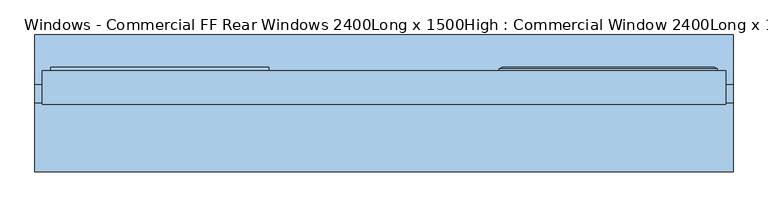
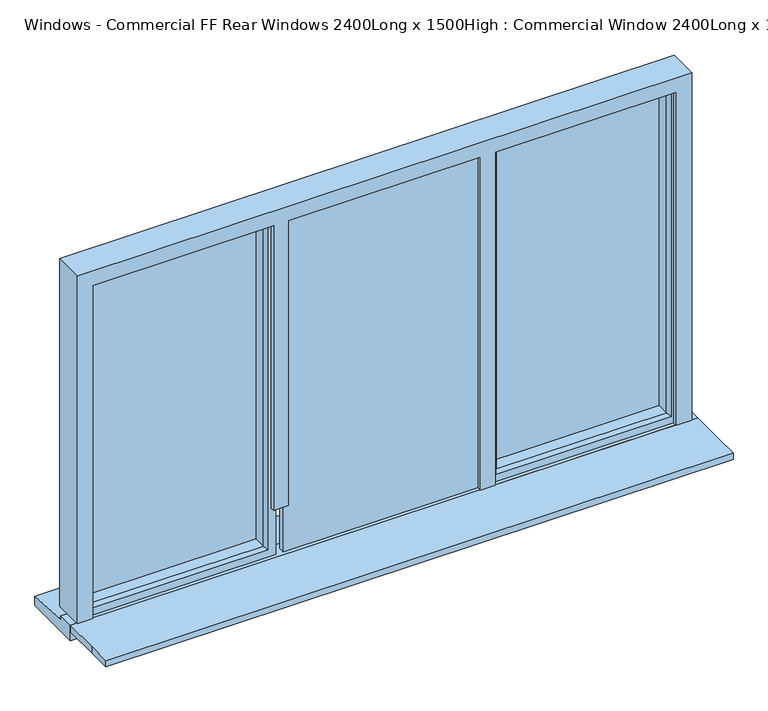
"""IFC4 building model written with IfcOpenShell, lengths in millimetres: window geometry, Windows - Commercial FF Rear Windows 2400Long x 1500High : Commercial Window 2400Long x 1500High."""

import ifcopenshell
import ifcopenshell.guid

model = None  # the IFC model being written
_history = None  # IfcOwnerHistory: only IFC2X3 demands one
_inside = {}  # id of a spatial element -> (the spatial element, [elements in it])
_under = {}  # id of a project, library or spatial element -> (it, [spatial elements below it])
_declared = {}  # id of a project -> (the project, [libraries it declares])
_typed = {}  # id of a type object -> (the type object, [elements of that type])
_made_of = {}  # id of a material, layer set ... -> (it, [elements and type objects made of it])


def new_model(schema):
    """Start an empty IFC model of exactly this schema.

    Asked for "IFC4X3", IfcOpenShell would pick the latest addendum, in which some entities
    have other attributes; the version numbers below select the first issue.
    IFC2X3 requires an IfcOwnerHistory on every rooted entity: one is made here for all.
    """
    global model, _history
    if schema == "IFC4X3":
        model = ifcopenshell.file(schema_version=(4, 3, 0, 0))
    else:
        model = ifcopenshell.file(schema=schema)
    _inside.clear()
    _under.clear()
    _declared.clear()
    _typed.clear()
    _made_of.clear()
    _history = None
    if model.schema == "IFC2X3":
        org = make("IfcOrganization", Name="unknown")
        user = make(
            "IfcPersonAndOrganization",
            ThePerson=make("IfcPerson", FamilyName="unknown"),
            TheOrganization=org,
        )
        app = make(
            "IfcApplication",
            ApplicationDeveloper=org,
            Version="unknown",
            ApplicationFullName="unknown",
            ApplicationIdentifier="unknown",
        )
        _history = make(
            "IfcOwnerHistory",
            OwningUser=user,
            OwningApplication=app,
            ChangeAction="ADDED",
            CreationDate=0,
        )
    return model


def make(cls, **values):
    """One entity of the class cls with the attributes given. An attribute that is None is left unset."""
    return model.create_entity(
        cls, **{name: value for name, value in values.items() if value is not None}
    )


def rooted(cls, **values):
    """An entity with a GlobalId (a new one), such as an element, a storey or a relation."""
    return make(cls, GlobalId=ifcopenshell.guid.new(), OwnerHistory=_history, **values)


def si_unit(unit_type, name, prefix=None):
    """IfcSIUnit, for example si_unit("LENGTHUNIT", "METRE", prefix="MILLI")."""
    return make("IfcSIUnit", UnitType=unit_type, Prefix=prefix, Name=name)


def assignment(units):
    """IfcUnitAssignment: the units of a project."""
    return None if units is None else make("IfcUnitAssignment", Units=units)


def point(xyz):
    """IfcCartesianPoint."""
    return None if xyz is None else make("IfcCartesianPoint", Coordinates=xyz)


def direction(xyz):
    """IfcDirection."""
    return None if xyz is None else make("IfcDirection", DirectionRatios=xyz)


def frame(location, z_axis=None, x_axis=None):
    """IfcAxis2Placement3D, a coordinate frame: its origin and axes. An axis left out is left unset."""
    return make(
        "IfcAxis2Placement3D",
        Location=point(location),
        Axis=direction(z_axis),
        RefDirection=direction(x_axis),
    )


def origin():
    """The frame at (0, 0, 0) with its axes left unset."""
    return frame((0.0, 0.0, 0.0))


def place(relative_to, where):
    """IfcLocalPlacement: puts the frame where relative to a parent placement (None: the world)."""
    return make(
        "IfcLocalPlacement", PlacementRelTo=relative_to, RelativePlacement=where
    )


def context(
    kind, dimensions, precision=None, world=None, true_north=None, identifier=None
):
    """IfcGeometricRepresentationContext, for example the 3D "Model" context."""
    return make(
        "IfcGeometricRepresentationContext",
        ContextIdentifier=identifier,
        ContextType=kind,
        CoordinateSpaceDimension=dimensions,
        Precision=precision,
        WorldCoordinateSystem=world,
        TrueNorth=true_north,
    )


def project(units=None, contexts=None):
    """IfcProject with its units and contexts."""
    return rooted(
        "IfcProject",
        Name="project",
        RepresentationContexts=contexts,
        UnitsInContext=assignment(units),
    )


def spatial(cls, under=None, at=None, **own):
    """A site, building, storey or space (cls), placed at a placement, below another one or the project."""
    s = rooted(cls, ObjectPlacement=at, **own)
    if under is not None:
        _under.setdefault(under.id(), (under, []))[1].append(s)
    return s


def polyline(points):
    """IfcPolyline through the points."""
    return make("IfcPolyline", Points=[point(p) for p in points])


def outline(outer, holes=None, kind="AREA"):
    """IfcArbitraryClosedProfileDef: a profile drawn as a closed curve; with holes, ...WithVoids."""
    if holes is None:
        return make("IfcArbitraryClosedProfileDef", ProfileType=kind, OuterCurve=outer)
    return make(
        "IfcArbitraryProfileDefWithVoids",
        ProfileType=kind,
        OuterCurve=outer,
        InnerCurves=holes,
    )


def extrude(swept, where, along, depth):
    """IfcExtrudedAreaSolid: the profile swept, set in the frame where, extruded along a direction by depth."""
    return make(
        "IfcExtrudedAreaSolid",
        SweptArea=swept,
        Position=where,
        ExtrudedDirection=direction(along),
        Depth=depth,
    )


def faces_of(points, faces, orient=None, outer=None):
    """IfcFace entities. A face is a list of loops; a loop is a list of indices into points, from 0.

    orient and outer hold one flag for each loop. By default every Orientation is true, the
    first loop of a face is its IfcFaceOuterBound and the others are IfcFaceBound.
    """
    made = []
    for i, loops in enumerate(faces):
        bounds = []
        for j, loop in enumerate(loops):
            is_outer = j == 0 if outer is None else outer[i][j]
            bounds.append(
                make(
                    "IfcFaceOuterBound" if is_outer else "IfcFaceBound",
                    Bound=make("IfcPolyLoop", Polygon=[points[k] for k in loop]),
                    Orientation=True if orient is None else orient[i][j],
                )
            )
        made.append(make("IfcFace", Bounds=bounds))
    return made


def faceted_brep(points, faces, orient=None, outer=None, voids=None):
    """IfcFacetedBrep: a solid bounded by flat faces; with voids (closed shells), ...WithVoids."""
    shared = [point(p) for p in points]
    hull = make("IfcClosedShell", CfsFaces=faces_of(shared, faces, orient, outer))
    if voids is None:
        return make("IfcFacetedBrep", Outer=hull)
    return make(
        "IfcFacetedBrepWithVoids",
        Outer=hull,
        Voids=[
            make(cls, CfsFaces=faces_of(shared, fs, o, b)) for cls, fs, o, b in voids
        ],
    )


def shape(context_of_items, identifier, shape_type, items):
    """IfcShapeRepresentation: the items that make up one representation, for example the "Body"."""
    return make(
        "IfcShapeRepresentation",
        ContextOfItems=context_of_items,
        RepresentationIdentifier=identifier,
        RepresentationType=shape_type,
        Items=items,
    )


def source(mapping_origin, context_of_items, identifier, shape_type, items):
    """IfcRepresentationMap: a shape defined once, which mapped items show again and again."""
    return make(
        "IfcRepresentationMap",
        MappingOrigin=mapping_origin,
        MappedRepresentation=shape(context_of_items, identifier, shape_type, items),
    )


def transform(
    local_origin,
    x_axis=None,
    y_axis=None,
    z_axis=None,
    scale=None,
    scale2=None,
    scale3=None,
    uniform=True,
):
    """IfcCartesianTransformationOperator3D, or its non-uniform kind. x_axis, y_axis, z_axis: its Axis1, 2, 3."""
    if uniform:
        return make(
            "IfcCartesianTransformationOperator3D",
            Axis1=direction(x_axis),
            Axis2=direction(y_axis),
            LocalOrigin=point(local_origin),
            Scale=scale,
            Axis3=direction(z_axis),
        )
    return make(
        "IfcCartesianTransformationOperator3DnonUniform",
        Axis1=direction(x_axis),
        Axis2=direction(y_axis),
        LocalOrigin=point(local_origin),
        Scale=scale,
        Axis3=direction(z_axis),
        Scale2=scale2,
        Scale3=scale3,
    )


def mapped(mapping_source, mapping_target):
    """IfcMappedItem: shows the shape of a source again, moved by a transform."""
    return make(
        "IfcMappedItem", MappingSource=mapping_source, MappingTarget=mapping_target
    )


def made_of(thing, what):
    """Note that an element or type object is made of a material, layer set ...; save() writes the relation."""
    if what is not None:
        _made_of.setdefault(what.id(), (what, []))[1].append(thing)
    return thing


def element(
    cls,
    number,
    at=None,
    inside=None,
    cuts=None,
    type_object=None,
    material=None,
    context=None,
    identifier="Body",
    shape_type=None,
    held_by="IfcProductDefinitionShape",
    body=None,
    shapes=None,
    **own,
):
    """One element of the class cls, such as IfcWall. Its Tag is "e" and its number.

    at: its placement. inside: the storey or other place that contains it. cuts: it is an
    opening in that element (IfcRelVoidsElement). A single representation is given by context,
    identifier, shape_type and body (its items); several are given by shapes. held_by: the class
    of the entity that holds the representations. save() writes the other relations.
    """
    e = rooted(cls, Tag="e%d" % number, ObjectPlacement=at, **own)
    if body is not None:
        shapes = [shape(context, identifier, shape_type, body)]
    if shapes is not None:
        e.Representation = make(held_by, Representations=shapes)
    if inside is not None:
        _inside.setdefault(inside.id(), (inside, []))[1].append(e)
    if cuts is not None:
        rooted(
            "IfcRelVoidsElement", RelatingBuildingElement=cuts, RelatedOpeningElement=e
        )
    if type_object is not None:
        _typed.setdefault(type_object.id(), (type_object, []))[1].append(e)
    return made_of(e, material)


def aggregate(whole, parts):
    """IfcRelAggregates: a whole, such as a stair, and the parts it consists of."""
    return rooted("IfcRelAggregates", RelatingObject=whole, RelatedObjects=parts)


def save(model, path):
    """Write the relations noted so far, then the file.

    IfcRelAggregates (storeys below a building ...), IfcRelContainedInSpatialStructure (elements
    in a storey), IfcRelDefinesByType, IfcRelAssociatesMaterial and IfcRelDeclares: one each for
    every whole, place, type object, material and project.
    """
    for whole, parts in _under.values():
        aggregate(whole, parts)
    for where, things in _inside.values():
        rooted(
            "IfcRelContainedInSpatialStructure",
            RelatedElements=things,
            RelatingStructure=where,
        )
    for kind, things in _typed.values():
        rooted("IfcRelDefinesByType", RelatedObjects=things, RelatingType=kind)
    for what, things in _made_of.values():
        rooted("IfcRelAssociatesMaterial", RelatedObjects=things, RelatingMaterial=what)
    for by, libraries in _declared.values():
        rooted("IfcRelDeclares", RelatingContext=by, RelatedDefinitions=libraries)
    model.write(path)


def windows_commercial_ff_rear_windows_2400long_x_1500high_d88e899e(model_context):
    return source(origin(), model_context, "Body", "SolidModel", [
        extrude(outline(polyline([(-1860.0, -231.5434322), (-1860.0, -138.5434322), (-1860.0, 8.4565678), (590.0, 8.4565678), (590.0, -138.5434322), (590.0, -231.5434322), (-1860.0, -231.5434322)])), frame((0.0, 0.0, 636.5715519), z_axis=(0.0, 0.0, 1.0), x_axis=(1.0, 0.0, 0.0)), (0.0, 0.0, 1.0), 26.4284481),
        extrude(outline(polyline([(495.0, 87.4565678), (-190.0, 87.4565678), (-190.0, 111.4565678), (495.0, 111.4565678), (495.0, 87.4565678)])), frame((0.0, 0.0, 693.0), z_axis=(0.0, 0.0, 1.0), x_axis=(1.0, 0.0, 0.0)), (0.0, 0.0, 1.0), 1337.0),
        extrude(outline(polyline([(-1020.0, 47.4565678), (-250.0, 47.4565678), (-250.0, 23.4565678), (-1020.0, 23.4565678), (-1020.0, 47.4565678)])), frame((0.0, 0.0, 663.0), z_axis=(0.0, 0.0, 1.0), x_axis=(1.0, 0.0, 0.0)), (0.0, 0.0, 1.0), 1397.0),
        extrude(outline(polyline([(-1080.0, 87.4565678), (-1765.0, 87.4565678), (-1765.0, 111.4565678), (-1080.0, 111.4565678), (-1080.0, 87.4565678)])), frame((0.0, 0.0, 693.0), z_axis=(0.0, 0.0, 1.0), x_axis=(1.0, 0.0, 0.0)), (0.0, 0.0, 1.0), 1337.0),
        faceted_brep([(-1835.0, 5.4565678, 663.0), (-1775.0, 5.4565678, 663.0), (-1775.0, 5.4565678, 2040.0), (-1068.0, 5.4565678, 2040.0), (-1068.0, 5.4565678, 863.0), (-1010.0, 5.4565678, 863.0), (-1010.0, 5.4565678, 2040.0), (-260.0, 5.4565678, 2040.0), (-260.0, 5.4565678, 663.0), (-202.0, 5.4565678, 663.0), (-202.0, 5.4565678, 2040.0), (505.0, 5.4565678, 2040.0), (505.0, 5.4565678, 663.0), (565.0, 5.4565678, 663.0), (565.0, 5.4565678, 2100.0), (-1835.0, 5.4565678, 2100.0), (-1835.0, 123.4565678, 2100.0), (-1835.0, 123.4565678, 663.0), (-1835.0, 73.4565678, 663.0), (-1835.0, 8.4565678, 663.0), (-1795.0, 123.4565678, 663.0), (565.0, 123.4565678, 2100.0), (565.0, 123.4565678, 663.0), (525.0, 123.4565678, 663.0), (525.0, 123.4565678, 2060.0), (-220.0, 123.4565678, 2060.0), (-220.0, 123.4565678, 663.0), (-260.0, 123.4565678, 663.0), (-260.0, 123.4565678, 2060.0), (-1010.0, 123.4565678, 2060.0), (-1010.0, 123.4565678, 863.0), (-1050.0, 123.4565678, 863.0), (-1050.0, 123.4565678, 2060.0), (-1795.0, 123.4565678, 2060.0), (-1795.0, 23.4565678, 2060.0), (-1795.0, 23.4565678, 663.0), (-1795.0, 73.4565678, 663.0), (-1050.0, 23.4565678, 2060.0), (-1050.0, 23.4565678, 863.0), (-1068.0, 23.4565678, 863.0), (-1068.0, 23.4565678, 2040.0), (-1775.0, 23.4565678, 2040.0), (-1775.0, 23.4565678, 663.0), (525.0, 23.4565678, 2060.0), (525.0, 23.4565678, 663.0), (505.0, 23.4565678, 663.0), (505.0, 23.4565678, 2040.0), (-202.0, 23.4565678, 2040.0), (-202.0, 23.4565678, 663.0), (-220.0, 23.4565678, 663.0), (-220.0, 23.4565678, 2060.0), (-1010.0, 23.4565678, 863.0), (-1020.0, 23.4565678, 863.0), (-1020.0, 23.4565678, 2060.0), (-250.0, 23.4565678, 2060.0), (-250.0, 23.4565678, 663.0), (-260.0, 23.4565678, 663.0), (-260.0, 23.4565678, 2040.0), (-1010.0, 23.4565678, 2040.0), (-1775.0, 8.4565678, 663.0), (-1010.0, 47.4565678, 2060.0), (-260.0, 47.4565678, 2060.0), (-250.0, 47.4565678, 2060.0), (-1020.0, 47.4565678, 2060.0), (565.0, 8.4565678, 663.0), (565.0, 73.4565678, 663.0), (525.0, 73.4565678, 663.0), (505.0, 8.4565678, 663.0), (-1010.0, 47.4565678, 863.0), (-1020.0, 47.4565678, 863.0), (-250.0, 47.4565678, 663.0), (-260.0, 47.4565678, 663.0), (-260.0, 73.4565678, 663.0), (-220.0, 73.4565678, 663.0), (-202.0, 8.4565678, 663.0), (-260.0, 8.4565678, 663.0), (590.0, 248.4565678, 600.0), (590.0, 8.4565678, 600.0), (-1860.0, 8.4565678, 600.0), (-1860.0, 248.4565678, 600.0), (590.0, 248.4565678, 637.0666405), (-1860.0, 248.4565678, 637.0666405), (590.0, 73.4565678, 649.0962075), (-1860.0, 73.4565678, 649.0962075), (590.0, 8.4565678, 663.0), (590.0, 73.4565678, 663.0), (-1860.0, 73.4565678, 663.0), (-1860.0, 8.4565678, 663.0)], [[[0, 1, 2, 3, 4, 5, 6, 7, 8, 9, 10, 11, 12, 13, 14, 15]], [[0, 15, 16, 17, 18, 19]], [[20, 17, 16, 21, 22, 23, 24, 25, 26, 27, 28, 29, 30, 31, 32, 33]], [[20, 33, 34, 35, 36]], [[35, 34, 37, 38, 39, 40, 41, 42]], [[43, 44, 45, 46, 47, 48, 49, 50]], [[51, 52, 53, 54, 55, 56, 57, 58]], [[2, 1, 59, 42, 41]], [[15, 14, 21, 16]], [[34, 33, 32, 37]], [[24, 43, 50, 25]], [[60, 29, 28, 61, 62, 54, 53, 63]], [[2, 41, 40, 3]], [[46, 11, 10, 47]], [[6, 58, 57, 7]], [[14, 13, 64, 65, 22, 21]], [[24, 23, 66, 44, 43]], [[12, 11, 46, 45, 67]], [[5, 51, 58, 6]], [[39, 4, 3, 40]], [[31, 38, 37, 32]], [[68, 30, 29, 60]], [[69, 68, 60, 63]], [[52, 69, 63, 53]], [[62, 70, 55, 54]], [[70, 62, 61, 71]], [[71, 61, 28, 27, 72]], [[26, 25, 50, 49, 73]], [[10, 9, 74, 48, 47]], [[8, 7, 57, 56, 75]], [[76, 77, 78, 79]], [[80, 76, 79, 81]], [[82, 80, 81, 83]], [[84, 85, 65, 64]], [[86, 87, 19, 18]], [[72, 36, 35, 42, 59, 75, 56, 55, 70, 71]], [[66, 73, 49, 48, 74, 67, 45, 44]], [[17, 20, 36, 18]], [[1, 0, 19, 59]], [[23, 22, 65, 66]], [[13, 12, 67, 64]], [[51, 5, 4, 39, 38, 31, 30, 68, 69, 52]], [[27, 26, 73, 72]], [[9, 8, 75, 74]], [[84, 77, 76, 80, 82, 85]], [[87, 86, 83, 81, 79, 78]], [[85, 82, 83, 86, 18, 36, 72, 73, 66, 65]], [[77, 84, 64, 67, 74, 75, 59, 19, 87, 78]]]),
        faceted_brep([(-1050.0, 23.4565678, 2060.0), (-1050.0, 93.4565678, 2060.0), (-1795.0, 93.4565678, 2060.0), (-1795.0, 23.4565678, 2060.0), (-1090.0, 37.9494677, 2020.0), (-1079.8519623, 23.4565678, 2030.1480377), (-1765.1480377, 23.4565678, 2030.1480377), (-1755.0, 37.9494677, 2020.0), (-1090.0, 87.4565678, 2020.0), (-1755.0, 87.4565678, 2020.0), (-1080.0, 111.4565678, 2030.0), (-1080.0, 87.4565678, 2030.0), (-1765.0, 87.4565678, 2030.0), (-1765.0, 111.4565678, 2030.0), (-1090.0, 129.2300705, 2020.0), (-1090.0, 111.4565678, 2020.0), (-1755.0, 111.4565678, 2020.0), (-1755.0, 129.2300705, 2020.0), (-1071.1854344, 135.0035732, 2038.8145656), (-1773.8145656, 135.0035732, 2038.8145656), (-1795.0, 93.4565678, 663.0), (-1795.0, 23.4565678, 663.0), (-1765.1480377, 23.4565678, 692.8519623), (-1755.0, 37.9494677, 703.0), (-1755.0, 87.4565678, 703.0), (-1765.0, 87.4565678, 693.0), (-1765.0, 111.4565678, 693.0), (-1755.0, 111.4565678, 703.0), (-1755.0, 129.2300705, 703.0), (-1773.8145656, 135.0035732, 684.1854344), (-1050.0, 93.4565678, 663.0), (-1050.0, 23.4565678, 663.0), (-1079.8519623, 23.4565678, 692.8519623), (-1090.0, 37.9494677, 703.0), (-1090.0, 87.4565678, 703.0), (-1080.0, 87.4565678, 693.0), (-1080.0, 111.4565678, 693.0), (-1090.0, 111.4565678, 703.0), (-1090.0, 129.2300705, 703.0), (-1071.1854344, 135.0035732, 684.1854344), (-1040.0, 135.0035732, 653.0), (-1805.0, 135.0035732, 653.0), (-1805.0, 135.0035732, 2070.0), (-1040.0, 135.0035732, 2070.0), (-1040.0, 93.4565678, 2070.0), (-1805.0, 93.4565678, 2070.0), (-1805.0, 93.4565678, 653.0), (-1040.0, 93.4565678, 653.0)], [[[0, 1, 2, 3]], [[4, 5, 6, 7]], [[8, 4, 7, 9]], [[10, 11, 12, 13]], [[14, 15, 16, 17]], [[18, 14, 17, 19]], [[3, 2, 20, 21]], [[7, 6, 22, 23]], [[9, 7, 23, 24]], [[13, 12, 25, 26]], [[17, 16, 27, 28]], [[19, 17, 28, 29]], [[21, 20, 30, 31]], [[0, 3, 21, 31], [32, 22, 6, 5]], [[23, 22, 32, 33]], [[24, 23, 33, 34]], [[35, 25, 12, 11], [8, 9, 24, 34]], [[26, 25, 35, 36]], [[10, 13, 26, 36], [37, 27, 16, 15]], [[28, 27, 37, 38]], [[29, 28, 38, 39]], [[40, 41, 42, 43], [18, 19, 29, 39]], [[30, 1, 0, 31]], [[33, 32, 5, 4]], [[34, 33, 4, 8]], [[36, 35, 11, 10]], [[38, 37, 15, 14]], [[39, 38, 14, 18]], [[44, 43, 42, 45]], [[45, 42, 41, 46]], [[46, 41, 40, 47]], [[47, 40, 43, 44]], [[45, 46, 47, 44], [1, 30, 20, 2]]]),
        faceted_brep([(-230.0, 87.4565678, 2070.0), (-230.0, 129.2300705, 2070.0), (-230.0, 129.2300705, 653.0), (-230.0, 87.4565678, 653.0), (-220.0, 23.4565678, 2060.0), (-220.0, 87.4565678, 2060.0), (-220.0, 87.4565678, 663.0), (-220.0, 23.4565678, 663.0), (-180.0, 37.9494677, 2020.0), (-190.1480377, 23.4565678, 2030.1480377), (-190.1480377, 23.4565678, 692.8519623), (-180.0, 37.9494677, 703.0), (-180.0, 87.4565678, 2020.0), (-180.0, 87.4565678, 703.0), (-190.0, 111.4565678, 2030.0), (-190.0, 87.4565678, 2030.0), (-190.0, 87.4565678, 693.0), (-190.0, 111.4565678, 693.0), (-180.0, 129.2300705, 2020.0), (-180.0, 111.4565678, 2020.0), (-180.0, 111.4565678, 703.0), (-180.0, 129.2300705, 703.0), (-197.4457548, 135.0035732, 2037.4457548), (-197.4457548, 135.0035732, 685.5542452), (-219.2153903, 135.0035732, 2059.2153903), (-219.2153903, 135.0035732, 663.7846097), (535.0, 129.2300705, 653.0), (535.0, 87.4565678, 653.0), (525.0, 87.4565678, 663.0), (525.0, 23.4565678, 663.0), (495.1480377, 23.4565678, 692.8519623), (485.0, 37.9494677, 703.0), (485.0, 87.4565678, 703.0), (495.0, 87.4565678, 693.0), (495.0, 111.4565678, 693.0), (485.0, 111.4565678, 703.0), (485.0, 129.2300705, 703.0), (502.4457548, 135.0035732, 685.5542452), (524.2153903, 135.0035732, 663.7846097), (535.0, 129.2300705, 2070.0), (535.0, 87.4565678, 2070.0), (525.0, 87.4565678, 2060.0), (525.0, 23.4565678, 2060.0), (495.1480377, 23.4565678, 2030.1480377), (485.0, 37.9494677, 2020.0), (485.0, 87.4565678, 2020.0), (495.0, 87.4565678, 2030.0), (495.0, 111.4565678, 2030.0), (485.0, 111.4565678, 2020.0), (485.0, 129.2300705, 2020.0), (502.4457548, 135.0035732, 2037.4457548), (524.2153903, 135.0035732, 2059.2153903)], [[[0, 1, 2, 3]], [[4, 5, 6, 7]], [[8, 9, 10, 11]], [[12, 8, 11, 13]], [[14, 15, 16, 17]], [[18, 19, 20, 21]], [[22, 18, 21, 23]], [[1, 24, 25, 2]], [[3, 2, 26, 27]], [[7, 6, 28, 29]], [[11, 10, 30, 31]], [[13, 11, 31, 32]], [[17, 16, 33, 34]], [[21, 20, 35, 36]], [[23, 21, 36, 37]], [[2, 25, 38, 26]], [[27, 26, 39, 40]], [[29, 28, 41, 42]], [[31, 30, 43, 44]], [[32, 31, 44, 45]], [[34, 33, 46, 47]], [[36, 35, 48, 49]], [[37, 36, 49, 50]], [[26, 38, 51, 39]], [[40, 39, 1, 0]], [[42, 41, 5, 4]], [[7, 29, 42, 4], [9, 43, 30, 10]], [[44, 43, 9, 8]], [[45, 44, 8, 12]], [[15, 46, 33, 16], [13, 32, 45, 12]], [[47, 46, 15, 14]], [[17, 34, 47, 14], [19, 48, 35, 20]], [[49, 48, 19, 18]], [[50, 49, 18, 22]], [[24, 51, 38, 25], [23, 37, 50, 22]], [[39, 51, 24, 1]], [[3, 27, 40, 0], [5, 41, 28, 6]]]),
    ])


if __name__ == "__main__":
    model = new_model("IFC4")
    model_context = context("Model", 3, world=origin())
    ifc_project = project(units=[si_unit("LENGTHUNIT", "METRE", prefix="MILLI")], contexts=[model_context])
    site = spatial("IfcSite", under=ifc_project)
    building = spatial("IfcBuilding", under=site)
    placement = place(None, origin())
    windows_commercial_ff_rear_windows_2400long_x_1500high_shape = windows_commercial_ff_rear_windows_2400long_x_1500high_d88e899e(model_context)
    element("IfcWindow", 1, ObjectType="Windows - Commercial FF Rear Windows 2400Long x 1500High : Commercial Window 2400Long x 1500High", at=placement, inside=building, context=model_context, shape_type="MappedRepresentation", body=[
        mapped(windows_commercial_ff_rear_windows_2400long_x_1500high_shape, transform((0.0, 0.0, 0.0), x_axis=(1.0, 0.0, 0.0), y_axis=(0.0, 1.0, 0.0), z_axis=(0.0, 0.0, 1.0))),
    ])
    save(model, "model.ifc")

# Revit data of these elements
# Type "Windows - Commercial FF Rear Windows 2400Long x 1500High : Commercial Window 2400Long x 1500High"
#   Type Mark = "45"
#   Operation = "TriplePanelVertical"
#   Description = "Double Glazed First Floor Window"
#   Manufacturer = "aluminium Co"
#   Keynote = "L10"
#   Wrap Layers (Ext) from Ext = 100 mm
#   Wrap Layers (Int) from Ext = 177.5 mm
#   Window Board Projection = 25 mm
#   Window Board Extension = 25 mm
#   Visual Light Transmittance = 0.9
#   Solar Heat Gain Coefficient = 0.78
#   Rough Width = 2400 mm
#   Rough Height = 1500 mm
#   Height = 1500 mm
#   Width = 2400 mm
#   Heat Transfer Coefficient (U) = 3.6886 W/(m²·K)
#   Glazing Thickness = 24 mm
#   FrameOffset - External = 100 mm
#   Frame Depth = 100 mm
#   Default Head Height = 2500 mm
#   Cill Depth = 125 mm
#   Cavity Closer Width = 75 mm
#   Cavity Closer Offset from Ext = 115 mm
#   Cavity Closer Depth = 100 mm
#   Vis - Cavity Closers = yes
#   Define Thermal Properties by = 1
#   Material Trim = Window Frame
#   Material Glass = Glass
#   Material Frame = Window Frame
#   Construction Type Id = ""
#   Wall Closure = (empty or 0)
#   Analytic Construction = (empty or 0)
# Element 1 (IfcWindow, "Windows - Commercial FF Rear Windows 2400Long x 1500High : Commercial Window 2400Long x 1500High")
#   Materials on its faces: "Window Frame", "Glass"
# Materials
#   "Window Frame": class "Miscellaneous", colour RGB 249 249 249, transparency 0, Keynote = "L10"
#   "Glass": class "Glass", colour RGB 0 128 192, transparency 0.9, Description = "Soda Lime Glass", Cost = 0
